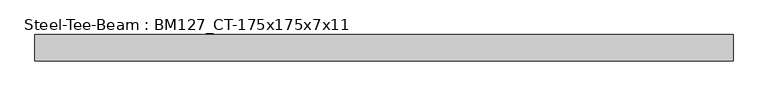
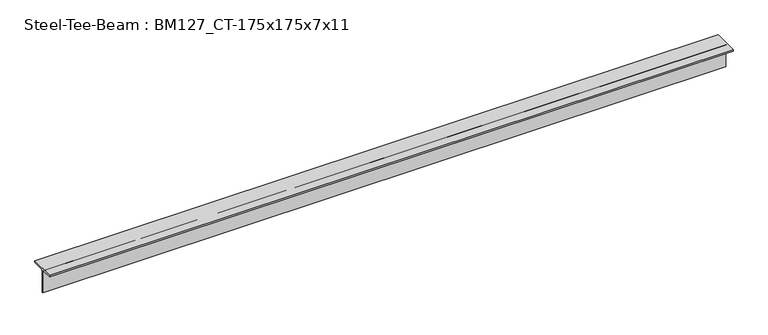
"""IFC4 building model written with IfcOpenShell, lengths in millimetres: beam geometry, Steel-Tee-Beam : BM127_CT-175x175x7x11."""

from ifc_helpers import new_model, si_unit, point, frame, frame_2d, origin, place, context, project, spatial, polyline, circle_curve, trimmed, segment, composite_curve, outline, extrude, source, transform, mapped, element, save


def steel_tee_beam_bm127_ct_175x175x7x11_4a9b7cbe(model_context):
    return source(origin(), model_context, "Body", "SweptSolid", [
        extrude(outline(composite_curve([segment(polyline([(-87.5, 87.5), (87.5, 87.5), (87.5, 76.5), (17.5, 76.5)]), True, "CONTINUOUS"), segment(trimmed(circle_curve(frame_2d((17.5, 62.5)), 14.0), [point((17.5, 76.5))], [point((3.5, 62.5))], True, "CARTESIAN"), True, "CONTINUOUS"), segment(polyline([(3.5, 62.5), (3.5, -87.5), (-3.5, -87.5), (-3.5, 62.5)]), True, "CONTINUOUS"), segment(trimmed(circle_curve(frame_2d((-17.5, 62.5)), 14.0), [point((-3.5, 62.5))], [point((-17.5, 76.5))], True, "CARTESIAN"), True, "CONTINUOUS"), segment(polyline([(-17.5, 76.5), (-87.5, 76.5), (-87.5, 87.5)]), True, "CONTINUOUS")], self_intersect=False)), frame((-2365.2579713, 0.0, 0.0), z_axis=(1.0, 0.0, 0.0), x_axis=(0.0, 1.0, 0.0)), (0.0, 0.0, 1.0), 4643.1263513),
    ])


if __name__ == "__main__":
    model = new_model("IFC4")
    model_context = context("Model", 3, world=origin())
    ifc_project = project(units=[si_unit("LENGTHUNIT", "METRE", prefix="MILLI")], contexts=[model_context])
    site = spatial("IfcSite", under=ifc_project)
    building = spatial("IfcBuilding", under=site)
    placement = place(None, origin())
    steel_tee_beam_bm127_ct_175x175x7x11_shape = steel_tee_beam_bm127_ct_175x175x7x11_4a9b7cbe(model_context)
    element("IfcBeam", 1, ObjectType="Steel-Tee-Beam : BM127_CT-175x175x7x11", at=placement, inside=building, context=model_context, shape_type="MappedRepresentation", body=[
        mapped(steel_tee_beam_bm127_ct_175x175x7x11_shape, transform((0.0, 0.0, 0.0), x_axis=(1.0, 0.0, 0.0), y_axis=(0.0, 1.0, 0.0), z_axis=(0.0, 0.0, 1.0))),
    ])
    save(model, "model.ifc")

# Revit data of these elements
# Type "Steel-Tee-Beam : BM127_CT-175x175x7x11"
#   Surface Area = 0.00 m²/m
#   Section Area = 31.57 cm²
#   Mass per Unit Length = 24.80 kg/m
#   Length [instance default] = 1524 mm
#   bf = 175 mm
#   d = 175 mm
#   k = 25 mm
#   kr = 14 mm
#   tf = 11 mm
#   tw = 7 mm
#   hec_material4 [instance default] = none
#   hec_material3 [instance default] = none
#   hec_material2 [instance default] = none
#   hec_material1 [instance default] = none
#   Structural Material [instance default] = Steel, 45-345
#   Assembly Code = ""
# Element 1 (IfcBeam, "Steel-Tee-Beam : BM127_CT-175x175x7x11")
#   hec_material3 = F01AC000-00002_Building/Shelter Fire Proofing Work_Intumescent Coating Type_1 hr. rating (UL 1709))
#   hec_material2 = S01AA010-00002_Main Steel Structure Fabrication Work_Shelter/Building_Steel Painting/Coating_for Fireproofed Steel Surface, Surface Preparation & Primer Coat
#   hec_material1 = S03AA029-00001_Main Steel Structure Erection Work_Shelter/Building_Light Steel
#   Structural Material = S01AA003-00001_Main Steel Structure Fabrication Work_Shelter/Building_Light Steel - Standard
#   Materials on its faces: "S01AA003-00001_Main Steel Structure Fabrication Work_Shelter/Building_Light Steel - Standard"
# Materials
#   "Steel, 45-345": class "Metal", colour RGB 189 187 185, transparency 0, Description = "Steel 345 MPa", Cost = 0
#   "S01AA003-00001_Main Steel Structure Fabrication Work_Shelter/Building_Light Steel - Standard": class "Metal", colour RGB 120 120 120, transparency 0, Comments = "(30KG/M>Weight)", Description = "Structural steel 50ksi", W00) Work Master Code = "S01AA003-00001", W01) Work Master_Lv1 = "Main Steel Structure Fabrication Work", W02) Work Master_Lv2 = "Shelter/Building", W03) Work Master_Spec.1 = "Light Steel - Standard (30KG/M>Weight)", Cost = 0
#   "F01AC000-00002_Building/Shelter Fire Proofing Work_Intumescent Coating Type_1 hr. rating (UL 1709))": class "Metal", colour RGB 255 128 128, transparency 0, Description = "Paint finished steel", W00) Work Master Code = "F01AC000-00002", W01) Work Master_Lv1 = "Building/Shelter Fire Proofing Work", W02) Work Master_Lv2 = "Intumescent Coating Type", W03) Work Master_Spec.1 = "1 hr. rating (UL 1709)", Cost = 0
#   "S01AA010-00002_Main Steel Structure Fabrication Work_Shelter/Building_Steel Painting/Coating_for Fireproofed Steel Surface, Surface Preparation & Primer Coat": class "Metal", colour RGB 120 120 120, transparency 0, Description = "Paint finished steel", W00) Work Master Code = "SS01AA010-00002", W01) Work Master_Lv1 = "Main Steel Structure Fabrication Work", W02) Work Master_Lv2 = "Shelter/Building", W03) Work Master_Spec.1 = "Steel Painting/Coating", W04) Work Master_Spec.2 = "for Fireproofed Steel Surface, Surface Preparation & Primer Coat", Cost = 0
#   "S03AA029-00001_Main Steel Structure Erection Work_Shelter/Building_Light Steel": class "Metal", colour RGB 120 120 120, transparency 0, Comments = "(30KG/M>Weight)", Description = "Structural steel 50ksi", W00) Work Master Code = "S03AA029-00001", W01) Work Master_Lv1 = "Main Steel Structure Erection Work", W02) Work Master_Lv2 = "Shelter/Building", W03) Work Master_Spec.1 = "Light Steel (30KG/M>Weight)", Cost = 0
